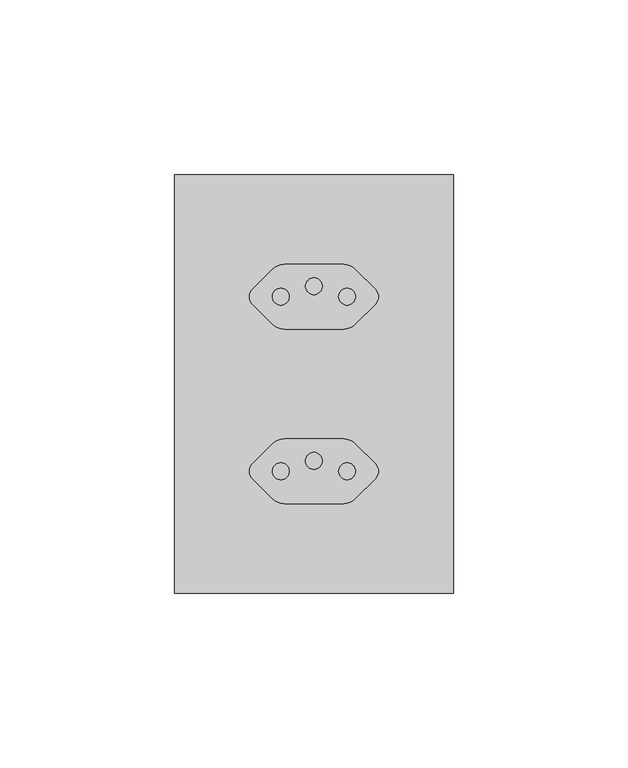
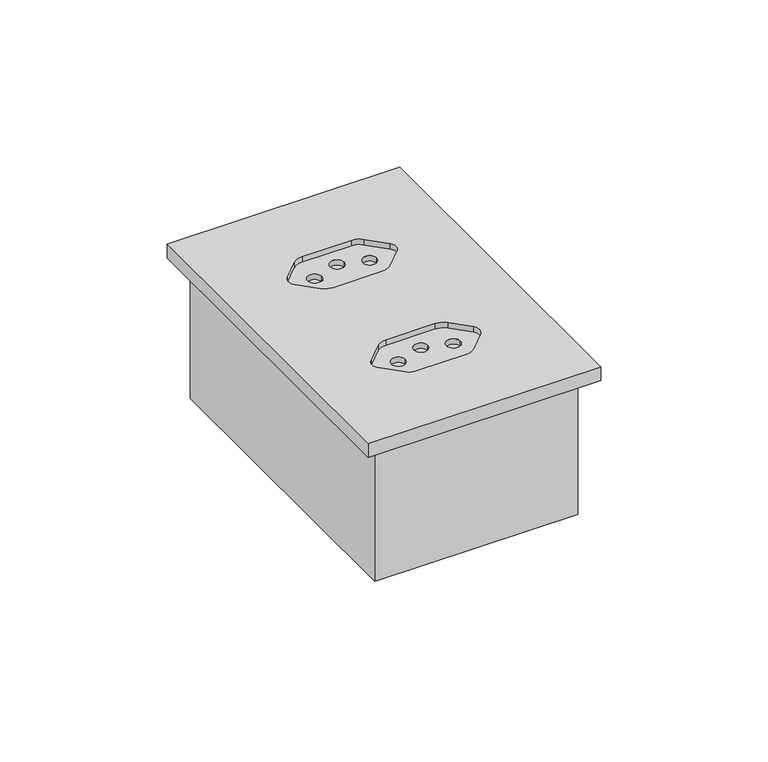
"""IFC4 building model written with IfcOpenShell, lengths in millimetres: proxy geometry, CAIXA VERTICE V7 : Tomada 20A 2s."""

from ifc_helpers import new_model, si_unit, frame, origin, place, context, project, spatial, polyline, circle_curve, faceted_brep, source, transform, mapped, element, save
from ifc_brep_helpers import plane_surface, revolved_surface, advanced_brep


def electrical_fixtures_e0bf078f(model_context):
    return source(origin(), model_context, "Body", "SolidModel", [
        faceted_brep([(33.0, 947.0, -48.0), (33.0, 1053.0, -48.0), (-33.0, 1053.0, -48.0), (-33.0, 947.0, -48.0), (35.0, 1055.0, -50.0), (35.0, 945.0, -50.0), (-35.0, 945.0, -50.0), (-35.0, 1055.0, -50.0), (-35.0, 1055.0, 0.0), (35.0, 1055.0, 0.0), (-35.0, 945.0, 0.0), (35.0, 945.0, 0.0), (33.0, 1053.0, 0.0), (33.0, 947.0, 0.0), (-33.0, 947.0, 0.0), (-33.0, 1053.0, 0.0)], [[[0, 1, 2, 3]], [[4, 5, 6, 7]], [[4, 7, 8, 9]], [[8, 7, 6, 10]], [[10, 6, 5, 11]], [[11, 5, 4, 9]], [[9, 8, 10, 11], [12, 13, 14, 15]], [[13, 12, 1, 0]], [[14, 13, 0, 3]], [[15, 14, 3, 2]], [[12, 15, 2, 1]]]),
        advanced_brep(
        [(40.0, 1060.0, 5.0), (-40.0, 1060.0, 5.0), (-40.0, 940.0, 5.0), (40.0, 940.0, 5.0), (8.4215729, 1015.75, 5.0), (-8.4215729, 1015.75, 5.0), (-11.9571068, 1017.2144661, 5.0), (-17.6213203, 1022.8786797, 5.0), (-17.6213203, 1027.1213203, 5.0), (-11.9571068, 1032.7855339, 5.0), (-8.4215729, 1034.25, 5.0), (8.4215729, 1034.25, 5.0), (11.9571068, 1032.7855339, 5.0), (17.6213203, 1027.1213203, 5.0), (17.6213203, 1022.8786797, 5.0), (11.9571068, 1017.2144661, 5.0), (8.4215729, 965.75, 5.0), (-8.4215729, 965.75, 5.0), (-11.9571068, 967.2144661, 5.0), (-17.6213203, 972.8786797, 5.0), (-17.6213203, 977.1213203, 5.0), (-11.9571068, 982.7855339, 5.0), (-8.4215729, 984.25, 5.0), (8.4215729, 984.25, 5.0), (11.9571068, 982.7855339, 5.0), (17.6213203, 977.1213203, 5.0), (17.6213203, 972.8786797, 5.0), (11.9571068, 967.2144661, 5.0), (-40.0, 1060.0, 0.0), (40.0, 1060.0, 0.0), (40.0, 940.0, 0.0), (-40.0, 940.0, 0.0), (8.4215729, 1015.75, 3.0), (11.9571068, 1017.2144661, 3.0), (17.6213203, 1022.8786797, 3.0), (17.6213203, 1027.1213203, 3.0), (11.9571068, 1032.7855339, 3.0), (8.4215729, 1034.25, 3.0), (-8.4215729, 1034.25, 3.0), (-11.9571068, 1032.7855339, 3.0), (-17.6213203, 1027.1213203, 3.0), (-17.6213203, 1022.8786797, 3.0), (-11.9571068, 1017.2144661, 3.0), (-8.4215729, 1015.75, 3.0), (-7.1, 1025.0, 3.0), (-11.9, 1025.0, 3.0), (11.9, 1025.0, 3.0), (7.1, 1025.0, 3.0), (2.4, 1028.0, 3.0), (-2.4, 1028.0, 3.0), (-11.9, 1025.0, 1.0), (-7.1, 1025.0, 1.0), (7.1, 1025.0, 1.0), (11.9, 1025.0, 1.0), (-2.4, 1028.0, 1.0), (2.4, 1028.0, 1.0), (8.4215729, 965.75, 3.0), (11.9571068, 967.2144661, 3.0), (17.6213203, 972.8786797, 3.0), (17.6213203, 977.1213203, 3.0), (11.9571068, 982.7855339, 3.0), (8.4215729, 984.25, 3.0), (-8.4215729, 984.25, 3.0), (-11.9571068, 982.7855339, 3.0), (-17.6213203, 977.1213203, 3.0), (-17.6213203, 972.8786797, 3.0), (-11.9571068, 967.2144661, 3.0), (-8.4215729, 965.75, 3.0), (-7.1, 975.0, 3.0), (-11.9, 975.0, 3.0), (11.9, 975.0, 3.0), (7.1, 975.0, 3.0), (2.4, 978.0, 3.0), (-2.4, 978.0, 3.0), (-11.9, 975.0, 1.0), (-7.1, 975.0, 1.0), (7.1, 975.0, 1.0), (11.9, 975.0, 1.0), (-2.4, 978.0, 1.0), (2.4, 978.0, 1.0)],
        [
            (0, 1),
            (1, 2),
            (2, 3),
            (3, 0),
            (4, 5),
            (5, 6, circle_curve(frame((-8.4215729, 1020.75, 5.0), z_axis=(0.0, 0.0, -1.0), x_axis=(-1.0, 0.0, 0.0)), 5.0)),
            (6, 7),
            (7, 8, circle_curve(frame((-15.5, 1025.0, 5.0), z_axis=(0.0, 0.0, -1.0), x_axis=(-1.0, 0.0, 0.0)), 3.0)),
            (8, 9),
            (9, 10, circle_curve(frame((-8.4215729, 1029.25, 5.0), z_axis=(0.0, 0.0, -1.0), x_axis=(-1.0, 0.0, 0.0)), 5.0)),
            (10, 11),
            (11, 12, circle_curve(frame((8.4215729, 1029.25, 5.0), z_axis=(0.0, 0.0, -1.0), x_axis=(-1.0, 0.0, 0.0)), 5.0)),
            (12, 13),
            (13, 14, circle_curve(frame((15.5, 1025.0, 5.0), z_axis=(0.0, 0.0, -1.0), x_axis=(-1.0, 0.0, 0.0)), 3.0)),
            (14, 15),
            (15, 4, circle_curve(frame((8.4215729, 1020.75, 5.0), z_axis=(0.0, 0.0, -1.0), x_axis=(-1.0, 0.0, 0.0)), 5.0)),
            (16, 17),
            (17, 18, circle_curve(frame((-8.4215729, 970.75, 5.0), z_axis=(0.0, 0.0, -1.0), x_axis=(-1.0, 0.0, 0.0)), 5.0)),
            (18, 19),
            (19, 20, circle_curve(frame((-15.5, 975.0, 5.0), z_axis=(0.0, 0.0, -1.0), x_axis=(-1.0, 0.0, 0.0)), 3.0)),
            (20, 21),
            (21, 22, circle_curve(frame((-8.4215729, 979.25, 5.0), z_axis=(0.0, 0.0, -1.0), x_axis=(-1.0, 0.0, 0.0)), 5.0)),
            (22, 23),
            (23, 24, circle_curve(frame((8.4215729, 979.25, 5.0), z_axis=(0.0, 0.0, -1.0), x_axis=(-1.0, 0.0, 0.0)), 5.0)),
            (24, 25),
            (25, 26, circle_curve(frame((15.5, 975.0, 5.0), z_axis=(0.0, 0.0, -1.0), x_axis=(-1.0, 0.0, 0.0)), 3.0)),
            (26, 27),
            (27, 16, circle_curve(frame((8.4215729, 970.75, 5.0), z_axis=(0.0, 0.0, -1.0), x_axis=(-1.0, 0.0, 0.0)), 5.0)),
            (28, 29),
            (29, 30),
            (30, 31),
            (31, 28),
            (0, 29),
            (28, 1),
            (31, 2),
            (30, 3),
            (32, 33, circle_curve(frame((8.4215729, 1020.75, 3.0), z_axis=(0.0, 0.0, 1.0), x_axis=(-1.0, 0.0, 0.0)), 5.0)),
            (33, 34),
            (34, 35, circle_curve(frame((15.5, 1025.0, 3.0), z_axis=(0.0, 0.0, 1.0), x_axis=(-1.0, 0.0, 0.0)), 3.0)),
            (35, 36),
            (36, 37, circle_curve(frame((8.4215729, 1029.25, 3.0), z_axis=(0.0, 0.0, 1.0), x_axis=(-1.0, 0.0, 0.0)), 5.0)),
            (37, 38),
            (38, 39, circle_curve(frame((-8.4215729, 1029.25, 3.0), z_axis=(0.0, 0.0, 1.0), x_axis=(-1.0, 0.0, 0.0)), 5.0)),
            (39, 40),
            (40, 41, circle_curve(frame((-15.5, 1025.0, 3.0), z_axis=(0.0, 0.0, 1.0), x_axis=(-1.0, 0.0, 0.0)), 3.0)),
            (41, 42),
            (42, 43, circle_curve(frame((-8.4215729, 1020.75, 3.0), z_axis=(0.0, 0.0, 1.0), x_axis=(-1.0, 0.0, 0.0)), 5.0)),
            (43, 32),
            (44, 45, circle_curve(frame((-9.5, 1025.0, 3.0), z_axis=(0.0, 0.0, -1.0), x_axis=(1.0, 2.301812013077709e-12, 0.0)), 2.4)),
            (45, 44, circle_curve(frame((-9.5, 1025.0, 3.0), z_axis=(0.0, 0.0, -1.0), x_axis=(1.0, 2.301812013077709e-12, 0.0)), 2.4)),
            (46, 47, circle_curve(frame((9.5, 1025.0, 3.0), z_axis=(0.0, 0.0, -1.0), x_axis=(1.0, 2.301812013077709e-12, 0.0)), 2.4)),
            (47, 46, circle_curve(frame((9.5, 1025.0, 3.0), z_axis=(0.0, 0.0, -1.0), x_axis=(1.0, 2.301812013077709e-12, 0.0)), 2.4)),
            (48, 49, circle_curve(frame((0.0, 1028.0, 3.0), z_axis=(0.0, 0.0, -1.0), x_axis=(1.0, 2.301812013077709e-12, 0.0)), 2.4)),
            (49, 48, circle_curve(frame((0.0, 1028.0, 3.0), z_axis=(0.0, 0.0, -1.0), x_axis=(1.0, 2.301812013077709e-12, 0.0)), 2.4)),
            (43, 5),
            (4, 32),
            (42, 6),
            (41, 7),
            (40, 8),
            (39, 9),
            (38, 10),
            (37, 11),
            (36, 12),
            (35, 13),
            (34, 14),
            (33, 15),
            (50, 51, circle_curve(frame((-9.5, 1025.0, 1.0), z_axis=(0.0, 0.0, 1.0), x_axis=(1.0, 2.301812013077709e-12, 0.0)), 2.4)),
            (51, 50, circle_curve(frame((-9.5, 1025.0, 1.0), z_axis=(0.0, 0.0, 1.0), x_axis=(1.0, 2.301812013077709e-12, 0.0)), 2.4)),
            (52, 53, circle_curve(frame((9.5, 1025.0, 1.0), z_axis=(0.0, 0.0, 1.0), x_axis=(1.0, 2.301812013077709e-12, 0.0)), 2.4)),
            (53, 52, circle_curve(frame((9.5, 1025.0, 1.0), z_axis=(0.0, 0.0, 1.0), x_axis=(1.0, 2.301812013077709e-12, 0.0)), 2.4)),
            (54, 55, circle_curve(frame((0.0, 1028.0, 1.0), z_axis=(0.0, 0.0, 1.0), x_axis=(1.0, 2.301812013077709e-12, 0.0)), 2.4)),
            (55, 54, circle_curve(frame((0.0, 1028.0, 1.0), z_axis=(0.0, 0.0, 1.0), x_axis=(1.0, 2.301812013077709e-12, 0.0)), 2.4)),
            (44, 51),
            (50, 45),
            (46, 53),
            (52, 47),
            (48, 55),
            (54, 49),
            (56, 57, circle_curve(frame((8.4215729, 970.75, 3.0), z_axis=(0.0, 0.0, 1.0), x_axis=(-1.0, 0.0, 0.0)), 5.0)),
            (57, 58),
            (58, 59, circle_curve(frame((15.5, 975.0, 3.0), z_axis=(0.0, 0.0, 1.0), x_axis=(-1.0, 0.0, 0.0)), 3.0)),
            (59, 60),
            (60, 61, circle_curve(frame((8.4215729, 979.25, 3.0), z_axis=(0.0, 0.0, 1.0), x_axis=(-1.0, 0.0, 0.0)), 5.0)),
            (61, 62),
            (62, 63, circle_curve(frame((-8.4215729, 979.25, 3.0), z_axis=(0.0, 0.0, 1.0), x_axis=(-1.0, 0.0, 0.0)), 5.0)),
            (63, 64),
            (64, 65, circle_curve(frame((-15.5, 975.0, 3.0), z_axis=(0.0, 0.0, 1.0), x_axis=(-1.0, 0.0, 0.0)), 3.0)),
            (65, 66),
            (66, 67, circle_curve(frame((-8.4215729, 970.75, 3.0), z_axis=(0.0, 0.0, 1.0), x_axis=(-1.0, 0.0, 0.0)), 5.0)),
            (67, 56),
            (68, 69, circle_curve(frame((-9.5, 975.0, 3.0), z_axis=(0.0, 0.0, -1.0), x_axis=(1.0, 2.301812013077709e-12, 0.0)), 2.4)),
            (69, 68, circle_curve(frame((-9.5, 975.0, 3.0), z_axis=(0.0, 0.0, -1.0), x_axis=(1.0, 2.301812013077709e-12, 0.0)), 2.4)),
            (70, 71, circle_curve(frame((9.5, 975.0, 3.0), z_axis=(0.0, 0.0, -1.0), x_axis=(1.0, 2.301812013077709e-12, 0.0)), 2.4)),
            (71, 70, circle_curve(frame((9.5, 975.0, 3.0), z_axis=(0.0, 0.0, -1.0), x_axis=(1.0, 2.301812013077709e-12, 0.0)), 2.4)),
            (72, 73, circle_curve(frame((0.0, 978.0, 3.0), z_axis=(0.0, 0.0, -1.0), x_axis=(1.0, 2.301812013077709e-12, 0.0)), 2.4)),
            (73, 72, circle_curve(frame((0.0, 978.0, 3.0), z_axis=(0.0, 0.0, -1.0), x_axis=(1.0, 2.301812013077709e-12, 0.0)), 2.4)),
            (67, 17),
            (16, 56),
            (66, 18),
            (65, 19),
            (64, 20),
            (63, 21),
            (62, 22),
            (61, 23),
            (60, 24),
            (59, 25),
            (58, 26),
            (57, 27),
            (74, 75, circle_curve(frame((-9.5, 975.0, 1.0), z_axis=(0.0, 0.0, 1.0), x_axis=(1.0, 2.301812013077709e-12, 0.0)), 2.4)),
            (75, 74, circle_curve(frame((-9.5, 975.0, 1.0), z_axis=(0.0, 0.0, 1.0), x_axis=(1.0, 2.301812013077709e-12, 0.0)), 2.4)),
            (76, 77, circle_curve(frame((9.5, 975.0, 1.0), z_axis=(0.0, 0.0, 1.0), x_axis=(1.0, 2.301812013077709e-12, 0.0)), 2.4)),
            (77, 76, circle_curve(frame((9.5, 975.0, 1.0), z_axis=(0.0, 0.0, 1.0), x_axis=(1.0, 2.301812013077709e-12, 0.0)), 2.4)),
            (78, 79, circle_curve(frame((0.0, 978.0, 1.0), z_axis=(0.0, 0.0, 1.0), x_axis=(1.0, 2.301812013077709e-12, 0.0)), 2.4)),
            (79, 78, circle_curve(frame((0.0, 978.0, 1.0), z_axis=(0.0, 0.0, 1.0), x_axis=(1.0, 2.301812013077709e-12, 0.0)), 2.4)),
            (68, 75),
            (74, 69),
            (70, 77),
            (76, 71),
            (72, 79),
            (78, 73),
        ],
        [
            plane_surface(frame((-60.0, 1060.0, 5.0), z_axis=(0.0, 0.0, 1.0), x_axis=(-1.0, 0.0, 0.0))),
            plane_surface(frame((-60.0, 1060.0, 0.0), z_axis=(0.0, 0.0, -1.0), x_axis=(1.0, 0.0, 0.0))),
            plane_surface(frame((40.0, 1060.0, 5.0), z_axis=(0.0, 1.0, 0.0), x_axis=(0.0, 0.0, -1.0))),
            plane_surface(frame((-40.0, 1060.0, 5.0), z_axis=(-1.0, 0.0, 0.0), x_axis=(0.0, 0.0, -1.0))),
            plane_surface(frame((-40.0, 940.0, 5.0), z_axis=(0.0, -1.0, 0.0), x_axis=(0.0, 0.0, -1.0))),
            plane_surface(frame((40.0, 940.0, 5.0), z_axis=(1.0, 0.0, 0.0), x_axis=(0.0, 0.0, -1.0))),
            plane_surface(frame((3.4215729, 1020.75, 3.0), z_axis=(0.0, 0.0, 1.0), x_axis=(0.0, 1.0, 0.0))),
            plane_surface(frame((-8.4215729, 1015.75, 5.0), z_axis=(0.0, 1.0, 0.0), x_axis=(0.0, 0.0, -1.0))),
            revolved_surface(polyline([(-13.4215729, 1020.75, 5.0), (-13.4215729, 1020.75, 3.0)]), (-8.4215729, 1020.75, 3.0), (0.0, 0.0, 1.0)),
            plane_surface(frame((-17.6213203, 1022.8786797, 5.0), z_axis=(0.7071067811865045, 0.7071067811865905, 0.0), x_axis=(0.0, 0.0, -1.0))),
            revolved_surface(polyline([(-18.5, 1025.0, 5.0), (-18.5, 1025.0, 3.0)]), (-15.5, 1025.0, 3.0), (0.0, 0.0, 1.0)),
            plane_surface(frame((-11.9571068, 1032.7855339, 5.0), z_axis=(0.7071067811865515, -0.7071067811865437, 0.0), x_axis=(0.0, 0.0, -1.0))),
            revolved_surface(polyline([(-13.4215729, 1029.25, 5.0), (-13.4215729, 1029.25, 3.0)]), (-8.4215729, 1029.25, 3.0), (0.0, 0.0, 1.0)),
            plane_surface(frame((8.4215729, 1034.25, 5.0), z_axis=(0.0, -1.0, 0.0), x_axis=(0.0, 0.0, -1.0))),
            revolved_surface(polyline([(3.4215728999999993, 1029.25, 5.0), (3.4215728999999993, 1029.25, 3.0)]), (8.4215729, 1029.25, 3.0), (0.0, 0.0, 1.0)),
            plane_surface(frame((17.6213203, 1027.1213203, 5.0), z_axis=(-0.7071067811865307, -0.7071067811865643, 0.0), x_axis=(0.0, 0.0, -1.0))),
            revolved_surface(polyline([(12.5, 1025.0, 5.0), (12.5, 1025.0, 3.0)]), (15.5, 1025.0, 3.0), (0.0, 0.0, 1.0)),
            plane_surface(frame((11.9571068, 1017.2144661, 5.0), z_axis=(-0.7071067811865893, 0.7071067811865058, 0.0), x_axis=(0.0, 0.0, -1.0))),
            revolved_surface(polyline([(3.4215728999999993, 1020.75, 5.0), (3.4215728999999993, 1020.75, 3.0)]), (8.4215729, 1020.75, 3.0), (0.0, 0.0, 1.0)),
            plane_surface(frame((-7.1, 1025.0, 1.0), z_axis=(0.0, 0.0, 1.0), x_axis=(2.301812013077709e-12, -1.0, 0.0))),
            revolved_surface(polyline([(-7.1, 1025.0000000000055, 3.0), (-7.1, 1025.0000000000055, 1.0)]), (-9.5, 1025.0, 1.0), (0.0, 0.0, 1.0)),
            revolved_surface(polyline([(11.9, 1025.0000000000055, 3.0), (11.9, 1025.0000000000055, 1.0)]), (9.5, 1025.0, 5.0), (0.0, 0.0, 1.0)),
            revolved_surface(polyline([(2.4, 1028.0000000000055, 3.0), (2.4, 1028.0000000000055, 1.0)]), (0.0, 1028.0, 5.0), (0.0, 0.0, 1.0)),
            plane_surface(frame((3.4215729, 970.75, 3.0), z_axis=(0.0, 0.0, 1.0), x_axis=(0.0, 1.0, 0.0))),
            plane_surface(frame((-8.4215729, 965.75, 5.0), z_axis=(0.0, 1.0, 0.0), x_axis=(0.0, 0.0, -1.0))),
            revolved_surface(polyline([(-13.4215729, 970.75, 5.0), (-13.4215729, 970.75, 3.0)]), (-8.4215729, 970.75, 3.0), (0.0, 0.0, 1.0)),
            plane_surface(frame((-17.6213203, 972.8786797, 5.0), z_axis=(0.7071067811865045, 0.7071067811865905, 0.0), x_axis=(0.0, 0.0, -1.0))),
            revolved_surface(polyline([(-18.5, 975.0, 5.0), (-18.5, 975.0, 3.0)]), (-15.5, 975.0, 3.0), (0.0, 0.0, 1.0)),
            plane_surface(frame((-11.9571068, 982.7855339, 5.0), z_axis=(0.7071067811865515, -0.7071067811865437, 0.0), x_axis=(0.0, 0.0, -1.0))),
            revolved_surface(polyline([(-13.4215729, 979.25, 5.0), (-13.4215729, 979.25, 3.0)]), (-8.4215729, 979.25, 3.0), (0.0, 0.0, 1.0)),
            plane_surface(frame((8.4215729, 984.25, 5.0), z_axis=(0.0, -1.0, 0.0), x_axis=(0.0, 0.0, -1.0))),
            revolved_surface(polyline([(3.4215728999999993, 979.25, 5.0), (3.4215728999999993, 979.25, 3.0)]), (8.4215729, 979.25, 3.0), (0.0, 0.0, 1.0)),
            plane_surface(frame((17.6213203, 977.1213203, 5.0), z_axis=(-0.7071067811865307, -0.7071067811865643, 0.0), x_axis=(0.0, 0.0, -1.0))),
            revolved_surface(polyline([(12.5, 975.0, 5.0), (12.5, 975.0, 3.0)]), (15.5, 975.0, 3.0), (0.0, 0.0, 1.0)),
            plane_surface(frame((11.9571068, 967.2144661, 5.0), z_axis=(-0.7071067811865893, 0.7071067811865058, 0.0), x_axis=(0.0, 0.0, -1.0))),
            revolved_surface(polyline([(3.4215728999999993, 970.75, 5.0), (3.4215728999999993, 970.75, 3.0)]), (8.4215729, 970.75, 3.0), (0.0, 0.0, 1.0)),
            plane_surface(frame((-7.1, 975.0, 1.0), z_axis=(0.0, 0.0, 1.0), x_axis=(2.301812013077709e-12, -1.0, 0.0))),
            revolved_surface(polyline([(-7.1, 975.0000000000056, 3.0), (-7.1, 975.0000000000056, 1.0)]), (-9.5, 975.0, 1.0), (0.0, 0.0, 1.0)),
            revolved_surface(polyline([(11.9, 975.0000000000056, 3.0), (11.9, 975.0000000000056, 1.0)]), (9.5, 975.0, 5.0), (0.0, 0.0, 1.0)),
            revolved_surface(polyline([(2.4, 978.0000000000056, 3.0), (2.4, 978.0000000000056, 1.0)]), (0.0, 978.0, 5.0), (0.0, 0.0, 1.0)),
        ],
        [
            (0, [[1, 2, 3, 4], [5, 6, 7, 8, 9, 10, 11, 12, 13, 14, 15, 16], [17, 18, 19, 20, 21, 22, 23, 24, 25, 26, 27, 28]]),
            (1, [[29, 30, 31, 32]]),
            (2, [[-1, 33, -29, 34]]),
            (3, [[-2, -34, -32, 35]]),
            (4, [[-3, -35, -31, 36]]),
            (5, [[-4, -36, -30, -33]]),
            (6, [[37, 38, 39, 40, 41, 42, 43, 44, 45, 46, 47, 48], [49, 50], [51, 52], [53, 54]]),
            (7, [[-48, 55, -5, 56]]),
            (8, [[-47, 57, -6, -55]]),
            (9, [[-46, 58, -7, -57]]),
            (10, [[-45, 59, -8, -58]]),
            (11, [[-44, 60, -9, -59]]),
            (12, [[-43, 61, -10, -60]]),
            (13, [[-42, 62, -11, -61]]),
            (14, [[-41, 63, -12, -62]]),
            (15, [[-40, 64, -13, -63]]),
            (16, [[-39, 65, -14, -64]]),
            (17, [[-38, 66, -15, -65]]),
            (18, [[-37, -56, -16, -66]]),
            (19, [[67, 68]]),
            (19, [[69, 70]]),
            (19, [[71, 72]]),
            (20, [[-49, 73, -67, 74]]),
            (20, [[-50, -74, -68, -73]]),
            (21, [[-51, 75, -69, 76]]),
            (21, [[-52, -76, -70, -75]]),
            (22, [[-53, 77, -71, 78]]),
            (22, [[-54, -78, -72, -77]]),
            (23, [[79, 80, 81, 82, 83, 84, 85, 86, 87, 88, 89, 90], [91, 92], [93, 94], [95, 96]]),
            (24, [[-90, 97, -17, 98]]),
            (25, [[-89, 99, -18, -97]]),
            (26, [[-88, 100, -19, -99]]),
            (27, [[-87, 101, -20, -100]]),
            (28, [[-86, 102, -21, -101]]),
            (29, [[-85, 103, -22, -102]]),
            (30, [[-84, 104, -23, -103]]),
            (31, [[-83, 105, -24, -104]]),
            (32, [[-82, 106, -25, -105]]),
            (33, [[-81, 107, -26, -106]]),
            (34, [[-80, 108, -27, -107]]),
            (35, [[-79, -98, -28, -108]]),
            (36, [[109, 110]]),
            (36, [[111, 112]]),
            (36, [[113, 114]]),
            (37, [[-91, 115, -109, 116]]),
            (37, [[-92, -116, -110, -115]]),
            (38, [[-93, 117, -111, 118]]),
            (38, [[-94, -118, -112, -117]]),
            (39, [[-95, 119, -113, 120]]),
            (39, [[-96, -120, -114, -119]]),
        ],
    ),
    ])


if __name__ == "__main__":
    model = new_model("IFC4")
    model_context = context("Model", 3, world=origin())
    ifc_project = project(units=[si_unit("LENGTHUNIT", "METRE", prefix="MILLI")], contexts=[model_context])
    site = spatial("IfcSite", under=ifc_project)
    building = spatial("IfcBuilding", under=site)
    placement = place(None, origin())
    electrical_fixtures_shape = electrical_fixtures_e0bf078f(model_context)
    element("IfcBuildingElementProxy", 1, Name="CAIXA VERTICE V7 : Tomada 20A 2s", ObjectType="CAIXA VERTICE V7 : Tomada 20A 2s", at=placement, inside=building, context=model_context, shape_type="MappedRepresentation", body=[
        mapped(electrical_fixtures_shape, transform((0.0, 0.0, 0.0), x_axis=(1.0, 0.0, 0.0), y_axis=(0.0, 1.0, 0.0), z_axis=(0.0, 0.0, 1.0))),
    ])
    save(model, "model.ifc")

# Revit data of these elements
# Type "CAIXA VERTICE V7 : Tomada 20A 2s"
#   URL = "www.facebook.com/verticetreinamentos"
#   SEÇÃO [instance default] = ""
#   Rotação [instance default] = 0.00°
#   LARGURA DA TAMPA = 0.08 m
#   BORDA = 0.01 m
#   ALTURA DE INSTALAÇÃO [instance default] = 1.10 m
#   Distância Anotação [instance default] = 0.0015 m
#   ALTURA DA TAMPA = 0.12 m
#   Vertical [instance default] = yes
#   VER SEÇÃO [instance default] = no
#   SHADE ESQ [instance default] = no
#   SHADE DIR [instance default] = yes
#   HORIZONTAL [instance default] = no
#   ANDAR COM A LEGENDA [instance default] = 0
#   Material Tampa [instance default] = Plástico, branco opaco
#   Caixa = element 1798518
#   Anotação = element 1798532
#   Default Elevation = 0
# Element 1 (IfcBuildingElementProxy, "CAIXA VERTICE V7 : Tomada 20A 2s")
#   ALTURA DE INSTALAÇÃO = 1.00 m
#   Materials on its faces: "Plástico, branco opaco"
# Materials
#   "Plástico, branco opaco": class "Plástico", colour RGB 120 120 120, transparency 0, Description = "Plastic, generic, opaque white", Cost = 0
